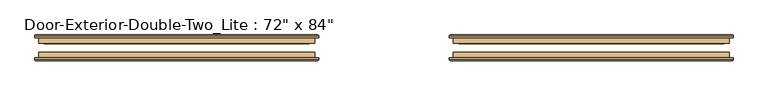
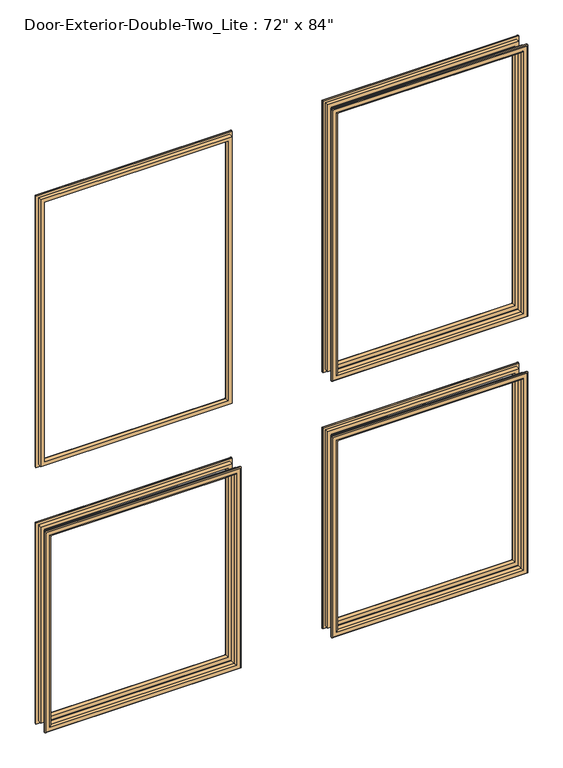
"""IFC4 building model written with IfcOpenShell, lengths in millimetres: door geometry."""

from ifc_helpers import new_model, si_unit, frame, origin, place, context, project, spatial, ellipse_curve, source, transform, mapped, element, save
from ifc_brep_helpers import plane_surface, cylinder_surface, advanced_brep


def door_5583bd1b(model_context):
    return source(origin(), model_context, "Body", "AdvancedBrep", [
        advanced_brep(
        [(-762.0, 55.5625, 914.4), (-762.0, 68.2625, 914.4), (-762.0, 68.2625, 254.0), (-762.0, 55.5625, 254.0), (-750.0, 69.2625, 902.4), (-750.0, 55.5625, 902.4), (-750.0, 55.5625, 266.0), (-750.0, 69.2625, 266.0), (-755.0, 74.2625, 907.4), (-755.0, 74.2625, 261.0), (-770.0, 72.2625, 922.4), (-768.0, 74.2625, 920.4), (-768.0, 74.2625, 248.0), (-770.0, 72.2625, 246.0), (-770.0, 68.2625, 922.4), (-770.0, 68.2625, 246.0), (-152.4, 68.2625, 254.0), (-152.4, 55.5625, 254.0), (-164.4, 55.5625, 266.0), (-164.4, 69.2625, 266.0), (-159.4, 74.2625, 261.0), (-146.4, 74.2625, 248.0), (-144.4, 72.2625, 246.0), (-144.4, 68.2625, 246.0), (-152.4, 68.2625, 914.4), (-152.4, 55.5625, 914.4), (-164.4, 55.5625, 902.4), (-164.4, 69.2625, 902.4), (-159.4, 74.2625, 907.4), (-146.4, 74.2625, 920.4), (-144.4, 72.2625, 922.4), (-144.4, 68.2625, 922.4)],
        [
            (0, 1),
            (1, 2),
            (2, 3),
            (3, 0),
            (4, 5),
            (5, 6),
            (6, 7),
            (7, 4),
            (8, 4, ellipse_curve(frame((-755.0, 69.2625, 907.4), z_axis=(-0.7071067811865475, 0.0, -0.7071067811865475), x_axis=(-0.7071067811865474, 0.0, 0.7071067811865476)), 7.0710678, 5.0)),
            (7, 9, ellipse_curve(frame((-755.0, 69.2625, 261.0), z_axis=(-0.7071067811865475, 0.0, 0.7071067811865475), x_axis=(0.7071067811865474, 0.0, 0.7071067811865476)), 7.0710678, 5.0)),
            (9, 8),
            (10, 11, ellipse_curve(frame((-768.0, 72.2625, 920.4), z_axis=(-0.7071067811865475, 0.0, -0.7071067811865475), x_axis=(-0.7071067811865474, 0.0, 0.7071067811865476)), 2.8284271, 2.0)),
            (11, 12),
            (12, 13, ellipse_curve(frame((-768.0, 72.2625, 248.0), z_axis=(-0.7071067811865475, 0.0, 0.7071067811865475), x_axis=(0.7071067811865474, 0.0, 0.7071067811865476)), 2.8284271, 2.0)),
            (13, 10),
            (14, 10),
            (13, 15),
            (15, 14),
            (2, 16),
            (16, 17),
            (17, 3),
            (6, 18),
            (18, 19),
            (19, 7),
            (19, 20, ellipse_curve(frame((-159.4, 69.2625, 261.0), z_axis=(-0.7071067811865475, 0.0, -0.7071067811865475), x_axis=(-0.7071067811865476, 0.0, 0.7071067811865474)), 7.0710678, 5.0)),
            (20, 9),
            (12, 21),
            (21, 22, ellipse_curve(frame((-146.4, 72.2625, 248.0), z_axis=(-0.7071067811865475, 0.0, -0.7071067811865475), x_axis=(-0.7071067811865476, 0.0, 0.7071067811865474)), 2.8284271, 2.0)),
            (22, 13),
            (22, 23),
            (23, 15),
            (16, 24),
            (24, 25),
            (25, 17),
            (18, 26),
            (26, 27),
            (27, 19),
            (27, 28, ellipse_curve(frame((-159.4, 69.2625, 907.4), z_axis=(0.7071067811865475, 0.0, -0.7071067811865475), x_axis=(-0.7071067811865474, 0.0, -0.7071067811865476)), 7.0710678, 5.0)),
            (28, 20),
            (21, 29),
            (29, 30, ellipse_curve(frame((-146.4, 72.2625, 920.4), z_axis=(0.7071067811865475, 0.0, -0.7071067811865475), x_axis=(-0.7071067811865474, 0.0, -0.7071067811865476)), 2.8284271, 2.0)),
            (30, 22),
            (30, 31),
            (31, 23),
            (31, 14),
            (1, 24),
            (0, 25),
            (5, 26),
            (4, 27),
            (8, 28),
            (11, 29),
            (10, 30),
        ],
        [
            plane_surface(frame((-762.0, 68.2625, 914.4), z_axis=(-1.0, 0.0, 0.0), x_axis=(0.0, 0.0, -1.0))),
            plane_surface(frame((-750.0, 55.5625, 902.4), z_axis=(1.0, 0.0, 0.0), x_axis=(0.0, 0.0, -1.0))),
            cylinder_surface(frame((-755.0, 69.2625, 914.4), z_axis=(0.0, 0.0, 1.0), x_axis=(-1.0, 0.0, 0.0)), 5.0),
            cylinder_surface(frame((-768.0, 72.2625, 914.4), z_axis=(0.0, 0.0, 1.0), x_axis=(-1.0, 0.0, 0.0)), 2.0),
            plane_surface(frame((-770.0, 72.2625, 922.4), z_axis=(-1.0, 0.0, 0.0), x_axis=(0.0, 0.0, -1.0))),
            plane_surface(frame((-762.0, 68.2625, 254.0), z_axis=(0.0, 0.0, -1.0), x_axis=(1.0, 0.0, 0.0))),
            plane_surface(frame((-750.0, 55.5625, 266.0), z_axis=(0.0, 0.0, 1.0), x_axis=(1.0, 0.0, 0.0))),
            cylinder_surface(frame((-762.0, 69.2625, 261.0), z_axis=(-1.0, 0.0, 0.0), x_axis=(0.0, 0.0, -1.0)), 5.0),
            cylinder_surface(frame((-762.0, 72.2625, 248.0), z_axis=(-1.0, 0.0, 0.0), x_axis=(0.0, 0.0, -1.0)), 2.0),
            plane_surface(frame((-770.0, 72.2625, 246.0), z_axis=(0.0, 0.0, -1.0), x_axis=(1.0, 0.0, 0.0))),
            plane_surface(frame((-152.4, 68.2625, 254.0), z_axis=(1.0, 0.0, 0.0), x_axis=(0.0, 0.0, 1.0))),
            plane_surface(frame((-164.4, 55.5625, 266.0), z_axis=(-1.0, 0.0, 0.0), x_axis=(0.0, 0.0, 1.0))),
            cylinder_surface(frame((-159.4, 69.2625, 254.0), z_axis=(0.0, 0.0, -1.0), x_axis=(1.0, 0.0, 0.0)), 5.0),
            cylinder_surface(frame((-146.4, 72.2625, 254.0), z_axis=(0.0, 0.0, -1.0), x_axis=(1.0, 0.0, 0.0)), 2.0),
            plane_surface(frame((-144.4, 72.2625, 246.0), z_axis=(1.0, 0.0, 0.0), x_axis=(0.0, 0.0, 1.0))),
            plane_surface(frame((-144.4, 68.2625, 922.4), z_axis=(0.0, -1.0, 0.0), x_axis=(-1.0, 0.0, 0.0))),
            plane_surface(frame((-152.4, 68.2625, 914.4), z_axis=(0.0, 0.0, 1.0), x_axis=(-1.0, 0.0, 0.0))),
            plane_surface(frame((-152.4, 55.5625, 914.4), z_axis=(0.0, -1.0, 0.0), x_axis=(-1.0, 0.0, 0.0))),
            plane_surface(frame((-164.4, 55.5625, 902.4), z_axis=(0.0, 0.0, -1.0), x_axis=(-1.0, 0.0, 0.0))),
            cylinder_surface(frame((-152.4, 69.2625, 907.4), z_axis=(1.0, 0.0, 0.0), x_axis=(0.0, 0.0, 1.0)), 5.0),
            plane_surface(frame((-159.4, 74.2625, 907.4), z_axis=(0.0, 1.0, 0.0), x_axis=(-1.0, 0.0, 0.0))),
            cylinder_surface(frame((-152.4, 72.2625, 920.4), z_axis=(1.0, 0.0, 0.0), x_axis=(0.0, 0.0, 1.0)), 2.0),
            plane_surface(frame((-144.4, 72.2625, 922.4), z_axis=(0.0, 0.0, 1.0), x_axis=(-1.0, 0.0, 0.0))),
        ],
        [
            (0, [[1, 2, 3, 4]]),
            (1, [[5, 6, 7, 8]]),
            (2, [[9, -8, 10, 11]]),
            (3, [[12, 13, 14, 15]]),
            (4, [[16, -15, 17, 18]]),
            (5, [[-3, 19, 20, 21]]),
            (6, [[-7, 22, 23, 24]]),
            (7, [[-10, -24, 25, 26]]),
            (8, [[-14, 27, 28, 29]]),
            (9, [[-17, -29, 30, 31]]),
            (10, [[-20, 32, 33, 34]]),
            (11, [[-23, 35, 36, 37]]),
            (12, [[-25, -37, 38, 39]]),
            (13, [[-28, 40, 41, 42]]),
            (14, [[-30, -42, 43, 44]]),
            (15, [[-31, -44, 45, -18], [46, -32, -19, -2]]),
            (16, [[-33, -46, -1, 47]]),
            (17, [[-21, -34, -47, -4], [48, -35, -22, -6]]),
            (18, [[-36, -48, -5, 49]]),
            (19, [[-38, -49, -9, 50]]),
            (20, [[51, -40, -27, -13], [-26, -39, -50, -11]]),
            (21, [[-41, -51, -12, 52]]),
            (22, [[-43, -52, -16, -45]]),
        ],
    ),
        advanced_brep(
        [(152.4, 55.5625, 914.4), (152.4, 68.2625, 914.4), (152.4, 68.2625, 254.0), (152.4, 55.5625, 254.0), (164.4, 69.2625, 902.4), (164.4, 55.5625, 902.4), (164.4, 55.5625, 266.0), (164.4, 69.2625, 266.0), (159.4, 74.2625, 907.4), (159.4, 74.2625, 261.0), (144.4, 72.2625, 922.4), (146.4, 74.2625, 920.4), (146.4, 74.2625, 248.0), (144.4, 72.2625, 246.0), (144.4, 68.2625, 922.4), (144.4, 68.2625, 246.0), (762.0, 68.2625, 254.0), (762.0, 55.5625, 254.0), (750.0, 55.5625, 266.0), (750.0, 69.2625, 266.0), (755.0, 74.2625, 261.0), (768.0, 74.2625, 248.0), (770.0, 72.2625, 246.0), (770.0, 68.2625, 246.0), (762.0, 68.2625, 914.4), (762.0, 55.5625, 914.4), (750.0, 55.5625, 902.4), (750.0, 69.2625, 902.4), (755.0, 74.2625, 907.4), (768.0, 74.2625, 920.4), (770.0, 72.2625, 922.4), (770.0, 68.2625, 922.4)],
        [
            (0, 1),
            (1, 2),
            (2, 3),
            (3, 0),
            (4, 5),
            (5, 6),
            (6, 7),
            (7, 4),
            (8, 4, ellipse_curve(frame((159.4, 69.2625, 907.4), z_axis=(-0.7071067811865475, 0.0, -0.7071067811865475), x_axis=(-0.7071067811865474, 0.0, 0.7071067811865476)), 7.0710678, 5.0)),
            (7, 9, ellipse_curve(frame((159.4, 69.2625, 261.0), z_axis=(-0.7071067811865475, 0.0, 0.7071067811865475), x_axis=(0.7071067811865474, 0.0, 0.7071067811865476)), 7.0710678, 5.0)),
            (9, 8),
            (10, 11, ellipse_curve(frame((146.4, 72.2625, 920.4), z_axis=(-0.7071067811865475, 0.0, -0.7071067811865475), x_axis=(-0.7071067811865474, 0.0, 0.7071067811865476)), 2.8284271, 2.0)),
            (11, 12),
            (12, 13, ellipse_curve(frame((146.4, 72.2625, 248.0), z_axis=(-0.7071067811865475, 0.0, 0.7071067811865475), x_axis=(0.7071067811865474, 0.0, 0.7071067811865476)), 2.8284271, 2.0)),
            (13, 10),
            (14, 10),
            (13, 15),
            (15, 14),
            (2, 16),
            (16, 17),
            (17, 3),
            (6, 18),
            (18, 19),
            (19, 7),
            (19, 20, ellipse_curve(frame((755.0, 69.2625, 261.0), z_axis=(-0.7071067811865475, 0.0, -0.7071067811865475), x_axis=(-0.7071067811865476, 0.0, 0.7071067811865474)), 7.0710678, 5.0)),
            (20, 9),
            (12, 21),
            (21, 22, ellipse_curve(frame((768.0, 72.2625, 248.0), z_axis=(-0.7071067811865475, 0.0, -0.7071067811865475), x_axis=(-0.7071067811865476, 0.0, 0.7071067811865474)), 2.8284271, 2.0)),
            (22, 13),
            (22, 23),
            (23, 15),
            (16, 24),
            (24, 25),
            (25, 17),
            (18, 26),
            (26, 27),
            (27, 19),
            (27, 28, ellipse_curve(frame((755.0, 69.2625, 907.4), z_axis=(0.7071067811865475, 0.0, -0.7071067811865475), x_axis=(-0.7071067811865474, 0.0, -0.7071067811865476)), 7.0710678, 5.0)),
            (28, 20),
            (21, 29),
            (29, 30, ellipse_curve(frame((768.0, 72.2625, 920.4), z_axis=(0.7071067811865475, 0.0, -0.7071067811865475), x_axis=(-0.7071067811865474, 0.0, -0.7071067811865476)), 2.8284271, 2.0)),
            (30, 22),
            (30, 31),
            (31, 23),
            (31, 14),
            (1, 24),
            (0, 25),
            (5, 26),
            (4, 27),
            (8, 28),
            (11, 29),
            (10, 30),
        ],
        [
            plane_surface(frame((152.4, 68.2625, 914.4), z_axis=(-1.0, 0.0, 0.0), x_axis=(0.0, 0.0, -1.0))),
            plane_surface(frame((164.4, 55.5625, 902.4), z_axis=(1.0, 0.0, 0.0), x_axis=(0.0, 0.0, -1.0))),
            cylinder_surface(frame((159.4, 69.2625, 914.4), z_axis=(0.0, 0.0, 1.0), x_axis=(-1.0, 0.0, 0.0)), 5.0),
            cylinder_surface(frame((146.4, 72.2625, 914.4), z_axis=(0.0, 0.0, 1.0), x_axis=(-1.0, 0.0, 0.0)), 2.0),
            plane_surface(frame((144.4, 72.2625, 922.4), z_axis=(-1.0, 0.0, 0.0), x_axis=(0.0, 0.0, -1.0))),
            plane_surface(frame((152.4, 68.2625, 254.0), z_axis=(0.0, 0.0, -1.0), x_axis=(1.0, 0.0, 0.0))),
            plane_surface(frame((164.4, 55.5625, 266.0), z_axis=(0.0, 0.0, 1.0), x_axis=(1.0, 0.0, 0.0))),
            cylinder_surface(frame((152.4, 69.2625, 261.0), z_axis=(-1.0, 0.0, 0.0), x_axis=(0.0, 0.0, -1.0)), 5.0),
            cylinder_surface(frame((152.4, 72.2625, 248.0), z_axis=(-1.0, 0.0, 0.0), x_axis=(0.0, 0.0, -1.0)), 2.0),
            plane_surface(frame((144.4, 72.2625, 246.0), z_axis=(0.0, 0.0, -1.0), x_axis=(1.0, 0.0, 0.0))),
            plane_surface(frame((762.0, 68.2625, 254.0), z_axis=(1.0, 0.0, 0.0), x_axis=(0.0, 0.0, 1.0))),
            plane_surface(frame((750.0, 55.5625, 266.0), z_axis=(-1.0, 0.0, 0.0), x_axis=(0.0, 0.0, 1.0))),
            cylinder_surface(frame((755.0, 69.2625, 254.0), z_axis=(0.0, 0.0, -1.0), x_axis=(1.0, 0.0, 0.0)), 5.0),
            cylinder_surface(frame((768.0, 72.2625, 254.0), z_axis=(0.0, 0.0, -1.0), x_axis=(1.0, 0.0, 0.0)), 2.0),
            plane_surface(frame((770.0, 72.2625, 246.0), z_axis=(1.0, 0.0, 0.0), x_axis=(0.0, 0.0, 1.0))),
            plane_surface(frame((770.0, 68.2625, 922.4), z_axis=(0.0, -1.0, 0.0), x_axis=(-1.0, 0.0, 0.0))),
            plane_surface(frame((762.0, 68.2625, 914.4), z_axis=(0.0, 0.0, 1.0), x_axis=(-1.0, 0.0, 0.0))),
            plane_surface(frame((762.0, 55.5625, 914.4), z_axis=(0.0, -1.0, 0.0), x_axis=(-1.0, 0.0, 0.0))),
            plane_surface(frame((750.0, 55.5625, 902.4), z_axis=(0.0, 0.0, -1.0), x_axis=(-1.0, 0.0, 0.0))),
            cylinder_surface(frame((762.0, 69.2625, 907.4), z_axis=(1.0, 0.0, 0.0), x_axis=(0.0, 0.0, 1.0)), 5.0),
            plane_surface(frame((755.0, 74.2625, 907.4), z_axis=(0.0, 1.0, 0.0), x_axis=(-1.0, 0.0, 0.0))),
            cylinder_surface(frame((762.0, 72.2625, 920.4), z_axis=(1.0, 0.0, 0.0), x_axis=(0.0, 0.0, 1.0)), 2.0),
            plane_surface(frame((770.0, 72.2625, 922.4), z_axis=(0.0, 0.0, 1.0), x_axis=(-1.0, 0.0, 0.0))),
        ],
        [
            (0, [[1, 2, 3, 4]]),
            (1, [[5, 6, 7, 8]]),
            (2, [[9, -8, 10, 11]]),
            (3, [[12, 13, 14, 15]]),
            (4, [[16, -15, 17, 18]]),
            (5, [[-3, 19, 20, 21]]),
            (6, [[-7, 22, 23, 24]]),
            (7, [[-10, -24, 25, 26]]),
            (8, [[-14, 27, 28, 29]]),
            (9, [[-17, -29, 30, 31]]),
            (10, [[-20, 32, 33, 34]]),
            (11, [[-23, 35, 36, 37]]),
            (12, [[-25, -37, 38, 39]]),
            (13, [[-28, 40, 41, 42]]),
            (14, [[-30, -42, 43, 44]]),
            (15, [[-31, -44, 45, -18], [46, -32, -19, -2]]),
            (16, [[-33, -46, -1, 47]]),
            (17, [[-21, -34, -47, -4], [48, -35, -22, -6]]),
            (18, [[-36, -48, -5, 49]]),
            (19, [[-38, -49, -9, 50]]),
            (20, [[51, -40, -27, -13], [-26, -39, -50, -11]]),
            (21, [[-41, -51, -12, 52]]),
            (22, [[-43, -52, -16, -45]]),
        ],
    ),
        advanced_brep(
        [(152.4, 55.5625, 2016.125), (152.4, 68.2625, 2016.125), (152.4, 68.2625, 1117.6), (152.4, 55.5625, 1117.6), (164.4, 69.2625, 2004.125), (164.4, 55.5625, 2004.125), (164.4, 55.5625, 1129.6), (164.4, 69.2625, 1129.6), (159.4, 74.2625, 2009.125), (159.4, 74.2625, 1124.6), (144.4, 72.2625, 2024.125), (146.4, 74.2625, 2022.125), (146.4, 74.2625, 1111.6), (144.4, 72.2625, 1109.6), (144.4, 68.2625, 2024.125), (144.4, 68.2625, 1109.6), (762.0, 68.2625, 1117.6), (762.0, 55.5625, 1117.6), (750.0, 55.5625, 1129.6), (750.0, 69.2625, 1129.6), (755.0, 74.2625, 1124.6), (768.0, 74.2625, 1111.6), (770.0, 72.2625, 1109.6), (770.0, 68.2625, 1109.6), (762.0, 68.2625, 2016.125), (762.0, 55.5625, 2016.125), (750.0, 55.5625, 2004.125), (750.0, 69.2625, 2004.125), (755.0, 74.2625, 2009.125), (768.0, 74.2625, 2022.125), (770.0, 72.2625, 2024.125), (770.0, 68.2625, 2024.125)],
        [
            (0, 1),
            (1, 2),
            (2, 3),
            (3, 0),
            (4, 5),
            (5, 6),
            (6, 7),
            (7, 4),
            (8, 4, ellipse_curve(frame((159.4, 69.2625, 2009.125), z_axis=(-0.7071067811865475, 0.0, -0.7071067811865475), x_axis=(-0.7071067811865474, 0.0, 0.7071067811865476)), 7.0710678, 5.0)),
            (7, 9, ellipse_curve(frame((159.4, 69.2625, 1124.6), z_axis=(-0.7071067811865475, 0.0, 0.7071067811865475), x_axis=(0.7071067811865474, 0.0, 0.7071067811865476)), 7.0710678, 5.0)),
            (9, 8),
            (10, 11, ellipse_curve(frame((146.4, 72.2625, 2022.125), z_axis=(-0.7071067811865475, 0.0, -0.7071067811865475), x_axis=(-0.7071067811865474, 0.0, 0.7071067811865476)), 2.8284271, 2.0)),
            (11, 12),
            (12, 13, ellipse_curve(frame((146.4, 72.2625, 1111.6), z_axis=(-0.7071067811865475, 0.0, 0.7071067811865475), x_axis=(0.7071067811865474, 0.0, 0.7071067811865476)), 2.8284271, 2.0)),
            (13, 10),
            (14, 10),
            (13, 15),
            (15, 14),
            (2, 16),
            (16, 17),
            (17, 3),
            (6, 18),
            (18, 19),
            (19, 7),
            (19, 20, ellipse_curve(frame((755.0, 69.2625, 1124.6), z_axis=(-0.7071067811865475, 0.0, -0.7071067811865475), x_axis=(-0.7071067811865476, 0.0, 0.7071067811865474)), 7.0710678, 5.0)),
            (20, 9),
            (12, 21),
            (21, 22, ellipse_curve(frame((768.0, 72.2625, 1111.6), z_axis=(-0.7071067811865475, 0.0, -0.7071067811865475), x_axis=(-0.7071067811865476, 0.0, 0.7071067811865474)), 2.8284271, 2.0)),
            (22, 13),
            (22, 23),
            (23, 15),
            (16, 24),
            (24, 25),
            (25, 17),
            (18, 26),
            (26, 27),
            (27, 19),
            (27, 28, ellipse_curve(frame((755.0, 69.2625, 2009.125), z_axis=(0.7071067811865475, 0.0, -0.7071067811865475), x_axis=(-0.7071067811865474, 0.0, -0.7071067811865476)), 7.0710678, 5.0)),
            (28, 20),
            (21, 29),
            (29, 30, ellipse_curve(frame((768.0, 72.2625, 2022.125), z_axis=(0.7071067811865475, 0.0, -0.7071067811865475), x_axis=(-0.7071067811865474, 0.0, -0.7071067811865476)), 2.8284271, 2.0)),
            (30, 22),
            (30, 31),
            (31, 23),
            (31, 14),
            (1, 24),
            (0, 25),
            (5, 26),
            (4, 27),
            (8, 28),
            (11, 29),
            (10, 30),
        ],
        [
            plane_surface(frame((152.4, 68.2625, 2016.125), z_axis=(-1.0, 0.0, 0.0), x_axis=(0.0, 0.0, -1.0))),
            plane_surface(frame((164.4, 55.5625, 2004.125), z_axis=(1.0, 0.0, 0.0), x_axis=(0.0, 0.0, -1.0))),
            cylinder_surface(frame((159.4, 69.2625, 2016.125), z_axis=(0.0, 0.0, 1.0), x_axis=(-1.0, 0.0, 0.0)), 5.0),
            cylinder_surface(frame((146.4, 72.2625, 2016.125), z_axis=(0.0, 0.0, 1.0), x_axis=(-1.0, 0.0, 0.0)), 2.0),
            plane_surface(frame((144.4, 72.2625, 2024.125), z_axis=(-1.0, 0.0, 0.0), x_axis=(0.0, 0.0, -1.0))),
            plane_surface(frame((152.4, 68.2625, 1117.6), z_axis=(0.0, 0.0, -1.0), x_axis=(1.0, 0.0, 0.0))),
            plane_surface(frame((164.4, 55.5625, 1129.6), z_axis=(0.0, 0.0, 1.0), x_axis=(1.0, 0.0, 0.0))),
            cylinder_surface(frame((152.4, 69.2625, 1124.6), z_axis=(-1.0, 0.0, 0.0), x_axis=(0.0, 0.0, -1.0)), 5.0),
            cylinder_surface(frame((152.4, 72.2625, 1111.6), z_axis=(-1.0, 0.0, 0.0), x_axis=(0.0, 0.0, -1.0)), 2.0),
            plane_surface(frame((144.4, 72.2625, 1109.6), z_axis=(0.0, 0.0, -1.0), x_axis=(1.0, 0.0, 0.0))),
            plane_surface(frame((762.0, 68.2625, 1117.6), z_axis=(1.0, 0.0, 0.0), x_axis=(0.0, 0.0, 1.0))),
            plane_surface(frame((750.0, 55.5625, 1129.6), z_axis=(-1.0, 0.0, 0.0), x_axis=(0.0, 0.0, 1.0))),
            cylinder_surface(frame((755.0, 69.2625, 1117.6), z_axis=(0.0, 0.0, -1.0), x_axis=(1.0, 0.0, 0.0)), 5.0),
            cylinder_surface(frame((768.0, 72.2625, 1117.6), z_axis=(0.0, 0.0, -1.0), x_axis=(1.0, 0.0, 0.0)), 2.0),
            plane_surface(frame((770.0, 72.2625, 1109.6), z_axis=(1.0, 0.0, 0.0), x_axis=(0.0, 0.0, 1.0))),
            plane_surface(frame((770.0, 68.2625, 2024.125), z_axis=(0.0, -1.0, 0.0), x_axis=(-1.0, 0.0, 0.0))),
            plane_surface(frame((762.0, 68.2625, 2016.125), z_axis=(0.0, 0.0, 1.0), x_axis=(-1.0, 0.0, 0.0))),
            plane_surface(frame((762.0, 55.5625, 2016.125), z_axis=(0.0, -1.0, 0.0), x_axis=(-1.0, 0.0, 0.0))),
            plane_surface(frame((750.0, 55.5625, 2004.125), z_axis=(0.0, 0.0, -1.0), x_axis=(-1.0, 0.0, 0.0))),
            cylinder_surface(frame((762.0, 69.2625, 2009.125), z_axis=(1.0, 0.0, 0.0), x_axis=(0.0, 0.0, 1.0)), 5.0),
            plane_surface(frame((755.0, 74.2625, 2009.125), z_axis=(0.0, 1.0, 0.0), x_axis=(-1.0, 0.0, 0.0))),
            cylinder_surface(frame((762.0, 72.2625, 2022.125), z_axis=(1.0, 0.0, 0.0), x_axis=(0.0, 0.0, 1.0)), 2.0),
            plane_surface(frame((770.0, 72.2625, 2024.125), z_axis=(0.0, 0.0, 1.0), x_axis=(-1.0, 0.0, 0.0))),
        ],
        [
            (0, [[1, 2, 3, 4]]),
            (1, [[5, 6, 7, 8]]),
            (2, [[9, -8, 10, 11]]),
            (3, [[12, 13, 14, 15]]),
            (4, [[16, -15, 17, 18]]),
            (5, [[-3, 19, 20, 21]]),
            (6, [[-7, 22, 23, 24]]),
            (7, [[-10, -24, 25, 26]]),
            (8, [[-14, 27, 28, 29]]),
            (9, [[-17, -29, 30, 31]]),
            (10, [[-20, 32, 33, 34]]),
            (11, [[-23, 35, 36, 37]]),
            (12, [[-25, -37, 38, 39]]),
            (13, [[-28, 40, 41, 42]]),
            (14, [[-30, -42, 43, 44]]),
            (15, [[-31, -44, 45, -18], [46, -32, -19, -2]]),
            (16, [[-33, -46, -1, 47]]),
            (17, [[-21, -34, -47, -4], [48, -35, -22, -6]]),
            (18, [[-36, -48, -5, 49]]),
            (19, [[-38, -49, -9, 50]]),
            (20, [[51, -40, -27, -13], [-26, -39, -50, -11]]),
            (21, [[-41, -51, -12, 52]]),
            (22, [[-43, -52, -16, -45]]),
        ],
    ),
        advanced_brep(
        [(-762.0, 55.5625, 2016.125), (-762.0, 68.2625, 2016.125), (-762.0, 68.2625, 1117.6), (-762.0, 55.5625, 1117.6), (-750.0, 69.2625, 2004.125), (-750.0, 55.5625, 2004.125), (-750.0, 55.5625, 1129.6), (-750.0, 69.2625, 1129.6), (-755.0, 74.2625, 2009.125), (-755.0, 74.2625, 1124.6), (-770.0, 72.2625, 2024.125), (-768.0, 74.2625, 2022.125), (-768.0, 74.2625, 1111.6), (-770.0, 72.2625, 1109.6), (-770.0, 68.2625, 2024.125), (-770.0, 68.2625, 1109.6), (-152.4, 68.2625, 1117.6), (-152.4, 55.5625, 1117.6), (-164.4, 55.5625, 1129.6), (-164.4, 69.2625, 1129.6), (-159.4, 74.2625, 1124.6), (-146.4, 74.2625, 1111.6), (-144.4, 72.2625, 1109.6), (-144.4, 68.2625, 1109.6), (-152.4, 68.2625, 2016.125), (-152.4, 55.5625, 2016.125), (-164.4, 55.5625, 2004.125), (-164.4, 69.2625, 2004.125), (-159.4, 74.2625, 2009.125), (-146.4, 74.2625, 2022.125), (-144.4, 72.2625, 2024.125), (-144.4, 68.2625, 2024.125)],
        [
            (0, 1),
            (1, 2),
            (2, 3),
            (3, 0),
            (4, 5),
            (5, 6),
            (6, 7),
            (7, 4),
            (8, 4, ellipse_curve(frame((-755.0, 69.2625, 2009.125), z_axis=(-0.7071067811865475, 0.0, -0.7071067811865475), x_axis=(-0.7071067811865474, 0.0, 0.7071067811865476)), 7.0710678, 5.0)),
            (7, 9, ellipse_curve(frame((-755.0, 69.2625, 1124.6), z_axis=(-0.7071067811865475, 0.0, 0.7071067811865475), x_axis=(0.7071067811865474, 0.0, 0.7071067811865476)), 7.0710678, 5.0)),
            (9, 8),
            (10, 11, ellipse_curve(frame((-768.0, 72.2625, 2022.125), z_axis=(-0.7071067811865475, 0.0, -0.7071067811865475), x_axis=(-0.7071067811865474, 0.0, 0.7071067811865476)), 2.8284271, 2.0)),
            (11, 12),
            (12, 13, ellipse_curve(frame((-768.0, 72.2625, 1111.6), z_axis=(-0.7071067811865475, 0.0, 0.7071067811865475), x_axis=(0.7071067811865474, 0.0, 0.7071067811865476)), 2.8284271, 2.0)),
            (13, 10),
            (14, 10),
            (13, 15),
            (15, 14),
            (2, 16),
            (16, 17),
            (17, 3),
            (6, 18),
            (18, 19),
            (19, 7),
            (19, 20, ellipse_curve(frame((-159.4, 69.2625, 1124.6), z_axis=(-0.7071067811865475, 0.0, -0.7071067811865475), x_axis=(-0.7071067811865476, 0.0, 0.7071067811865474)), 7.0710678, 5.0)),
            (20, 9),
            (12, 21),
            (21, 22, ellipse_curve(frame((-146.4, 72.2625, 1111.6), z_axis=(-0.7071067811865475, 0.0, -0.7071067811865475), x_axis=(-0.7071067811865476, 0.0, 0.7071067811865474)), 2.8284271, 2.0)),
            (22, 13),
            (22, 23),
            (23, 15),
            (16, 24),
            (24, 25),
            (25, 17),
            (18, 26),
            (26, 27),
            (27, 19),
            (27, 28, ellipse_curve(frame((-159.4, 69.2625, 2009.125), z_axis=(0.7071067811865475, 0.0, -0.7071067811865475), x_axis=(-0.7071067811865474, 0.0, -0.7071067811865476)), 7.0710678, 5.0)),
            (28, 20),
            (21, 29),
            (29, 30, ellipse_curve(frame((-146.4, 72.2625, 2022.125), z_axis=(0.7071067811865475, 0.0, -0.7071067811865475), x_axis=(-0.7071067811865474, 0.0, -0.7071067811865476)), 2.8284271, 2.0)),
            (30, 22),
            (30, 31),
            (31, 23),
            (31, 14),
            (1, 24),
            (0, 25),
            (5, 26),
            (4, 27),
            (8, 28),
            (11, 29),
            (10, 30),
        ],
        [
            plane_surface(frame((-762.0, 68.2625, 2016.125), z_axis=(-1.0, 0.0, 0.0), x_axis=(0.0, 0.0, -1.0))),
            plane_surface(frame((-750.0, 55.5625, 2004.125), z_axis=(1.0, 0.0, 0.0), x_axis=(0.0, 0.0, -1.0))),
            cylinder_surface(frame((-755.0, 69.2625, 2016.125), z_axis=(0.0, 0.0, 1.0), x_axis=(-1.0, 0.0, 0.0)), 5.0),
            cylinder_surface(frame((-768.0, 72.2625, 2016.125), z_axis=(0.0, 0.0, 1.0), x_axis=(-1.0, 0.0, 0.0)), 2.0),
            plane_surface(frame((-770.0, 72.2625, 2024.125), z_axis=(-1.0, 0.0, 0.0), x_axis=(0.0, 0.0, -1.0))),
            plane_surface(frame((-762.0, 68.2625, 1117.6), z_axis=(0.0, 0.0, -1.0), x_axis=(1.0, 0.0, 0.0))),
            plane_surface(frame((-750.0, 55.5625, 1129.6), z_axis=(0.0, 0.0, 1.0), x_axis=(1.0, 0.0, 0.0))),
            cylinder_surface(frame((-762.0, 69.2625, 1124.6), z_axis=(-1.0, 0.0, 0.0), x_axis=(0.0, 0.0, -1.0)), 5.0),
            cylinder_surface(frame((-762.0, 72.2625, 1111.6), z_axis=(-1.0, 0.0, 0.0), x_axis=(0.0, 0.0, -1.0)), 2.0),
            plane_surface(frame((-770.0, 72.2625, 1109.6), z_axis=(0.0, 0.0, -1.0), x_axis=(1.0, 0.0, 0.0))),
            plane_surface(frame((-152.4, 68.2625, 1117.6), z_axis=(1.0, 0.0, 0.0), x_axis=(0.0, 0.0, 1.0))),
            plane_surface(frame((-164.4, 55.5625, 1129.6), z_axis=(-1.0, 0.0, 0.0), x_axis=(0.0, 0.0, 1.0))),
            cylinder_surface(frame((-159.4, 69.2625, 1117.6), z_axis=(0.0, 0.0, -1.0), x_axis=(1.0, 0.0, 0.0)), 5.0),
            cylinder_surface(frame((-146.4, 72.2625, 1117.6), z_axis=(0.0, 0.0, -1.0), x_axis=(1.0, 0.0, 0.0)), 2.0),
            plane_surface(frame((-144.4, 72.2625, 1109.6), z_axis=(1.0, 0.0, 0.0), x_axis=(0.0, 0.0, 1.0))),
            plane_surface(frame((-144.4, 68.2625, 2024.125), z_axis=(0.0, -1.0, 0.0), x_axis=(-1.0, 0.0, 0.0))),
            plane_surface(frame((-152.4, 68.2625, 2016.125), z_axis=(0.0, 0.0, 1.0), x_axis=(-1.0, 0.0, 0.0))),
            plane_surface(frame((-152.4, 55.5625, 2016.125), z_axis=(0.0, -1.0, 0.0), x_axis=(-1.0, 0.0, 0.0))),
            plane_surface(frame((-164.4, 55.5625, 2004.125), z_axis=(0.0, 0.0, -1.0), x_axis=(-1.0, 0.0, 0.0))),
            cylinder_surface(frame((-152.4, 69.2625, 2009.125), z_axis=(1.0, 0.0, 0.0), x_axis=(0.0, 0.0, 1.0)), 5.0),
            plane_surface(frame((-159.4, 74.2625, 2009.125), z_axis=(0.0, 1.0, 0.0), x_axis=(-1.0, 0.0, 0.0))),
            cylinder_surface(frame((-152.4, 72.2625, 2022.125), z_axis=(1.0, 0.0, 0.0), x_axis=(0.0, 0.0, 1.0)), 2.0),
            plane_surface(frame((-144.4, 72.2625, 2024.125), z_axis=(0.0, 0.0, 1.0), x_axis=(-1.0, 0.0, 0.0))),
        ],
        [
            (0, [[1, 2, 3, 4]]),
            (1, [[5, 6, 7, 8]]),
            (2, [[9, -8, 10, 11]]),
            (3, [[12, 13, 14, 15]]),
            (4, [[16, -15, 17, 18]]),
            (5, [[-3, 19, 20, 21]]),
            (6, [[-7, 22, 23, 24]]),
            (7, [[-10, -24, 25, 26]]),
            (8, [[-14, 27, 28, 29]]),
            (9, [[-17, -29, 30, 31]]),
            (10, [[-20, 32, 33, 34]]),
            (11, [[-23, 35, 36, 37]]),
            (12, [[-25, -37, 38, 39]]),
            (13, [[-28, 40, 41, 42]]),
            (14, [[-30, -42, 43, 44]]),
            (15, [[-31, -44, 45, -18], [46, -32, -19, -2]]),
            (16, [[-33, -46, -1, 47]]),
            (17, [[-21, -34, -47, -4], [48, -35, -22, -6]]),
            (18, [[-36, -48, -5, 49]]),
            (19, [[-38, -49, -9, 50]]),
            (20, [[51, -40, -27, -13], [-26, -39, -50, -11]]),
            (21, [[-41, -51, -12, 52]]),
            (22, [[-43, -52, -16, -45]]),
        ],
    ),
        advanced_brep(
        [(-762.0, 36.5125, 254.0), (-762.0, 23.8125, 254.0), (-762.0, 23.8125, 914.4), (-762.0, 36.5125, 914.4), (-750.0, 22.8125, 266.0), (-750.0, 36.5125, 266.0), (-750.0, 36.5125, 902.4), (-750.0, 22.8125, 902.4), (-755.0, 17.8125, 261.0), (-755.0, 17.8125, 907.4), (-770.0, 19.8125, 246.0), (-768.0, 17.8125, 248.0), (-768.0, 17.8125, 920.4), (-770.0, 19.8125, 922.4), (-770.0, 23.8125, 246.0), (-770.0, 23.8125, 922.4), (-152.4, 23.8125, 914.4), (-152.4, 36.5125, 914.4), (-164.4, 36.5125, 902.4), (-164.4, 22.8125, 902.4), (-159.4, 17.8125, 907.4), (-146.4, 17.8125, 920.4), (-144.4, 19.8125, 922.4), (-144.4, 23.8125, 922.4), (-152.4, 23.8125, 254.0), (-152.4, 36.5125, 254.0), (-164.4, 36.5125, 266.0), (-164.4, 22.8125, 266.0), (-159.4, 17.8125, 261.0), (-146.4, 17.8125, 248.0), (-144.4, 19.8125, 246.0), (-144.4, 23.8125, 246.0)],
        [
            (0, 1),
            (1, 2),
            (2, 3),
            (3, 0),
            (4, 5),
            (5, 6),
            (6, 7),
            (7, 4),
            (8, 4, ellipse_curve(frame((-755.0, 22.8125, 261.0), z_axis=(-0.7071067811865475, 0.0, 0.7071067811865475), x_axis=(-0.7071067811865474, 0.0, -0.7071067811865476)), 7.0710678, 5.0)),
            (7, 9, ellipse_curve(frame((-755.0, 22.8125, 907.4), z_axis=(-0.7071067811865475, 0.0, -0.7071067811865475), x_axis=(0.7071067811865474, 0.0, -0.7071067811865476)), 7.0710678, 5.0)),
            (9, 8),
            (10, 11, ellipse_curve(frame((-768.0, 19.8125, 248.0), z_axis=(-0.7071067811865475, 0.0, 0.7071067811865475), x_axis=(-0.7071067811865474, 0.0, -0.7071067811865476)), 2.8284271, 2.0)),
            (11, 12),
            (12, 13, ellipse_curve(frame((-768.0, 19.8125, 920.4), z_axis=(-0.7071067811865475, 0.0, -0.7071067811865475), x_axis=(0.7071067811865474, 0.0, -0.7071067811865476)), 2.8284271, 2.0)),
            (13, 10),
            (14, 10),
            (13, 15),
            (15, 14),
            (2, 16),
            (16, 17),
            (17, 3),
            (6, 18),
            (18, 19),
            (19, 7),
            (19, 20, ellipse_curve(frame((-159.4, 22.8125, 907.4), z_axis=(-0.7071067811865475, 0.0, 0.7071067811865475), x_axis=(-0.7071067811865476, 0.0, -0.7071067811865474)), 7.0710678, 5.0)),
            (20, 9),
            (12, 21),
            (21, 22, ellipse_curve(frame((-146.4, 19.8125, 920.4), z_axis=(-0.7071067811865475, 0.0, 0.7071067811865475), x_axis=(-0.7071067811865476, 0.0, -0.7071067811865474)), 2.8284271, 2.0)),
            (22, 13),
            (22, 23),
            (23, 15),
            (16, 24),
            (24, 25),
            (25, 17),
            (18, 26),
            (26, 27),
            (27, 19),
            (27, 28, ellipse_curve(frame((-159.4, 22.8125, 261.0), z_axis=(0.7071067811865475, 0.0, 0.7071067811865475), x_axis=(-0.7071067811865474, 0.0, 0.7071067811865476)), 7.0710678, 5.0)),
            (28, 20),
            (21, 29),
            (29, 30, ellipse_curve(frame((-146.4, 19.8125, 248.0), z_axis=(0.7071067811865475, 0.0, 0.7071067811865475), x_axis=(-0.7071067811865474, 0.0, 0.7071067811865476)), 2.8284271, 2.0)),
            (30, 22),
            (30, 31),
            (31, 23),
            (31, 14),
            (1, 24),
            (0, 25),
            (5, 26),
            (4, 27),
            (8, 28),
            (11, 29),
            (10, 30),
        ],
        [
            plane_surface(frame((-762.0, 23.8125, 254.0), z_axis=(-1.0, 0.0, 0.0), x_axis=(0.0, 0.0, 1.0))),
            plane_surface(frame((-750.0, 36.5125, 266.0), z_axis=(1.0, 0.0, 0.0), x_axis=(0.0, 0.0, 1.0))),
            cylinder_surface(frame((-755.0, 22.8125, 254.0), z_axis=(0.0, 0.0, -1.0), x_axis=(-1.0, 0.0, 0.0)), 5.0),
            cylinder_surface(frame((-768.0, 19.8125, 254.0), z_axis=(0.0, 0.0, -1.0), x_axis=(-1.0, 0.0, 0.0)), 2.0),
            plane_surface(frame((-770.0, 19.8125, 246.0), z_axis=(-1.0, 0.0, 0.0), x_axis=(0.0, 0.0, 1.0))),
            plane_surface(frame((-762.0, 23.8125, 914.4), z_axis=(0.0, 0.0, 1.0), x_axis=(1.0, 0.0, 0.0))),
            plane_surface(frame((-750.0, 36.5125, 902.4), z_axis=(0.0, 0.0, -1.0), x_axis=(1.0, 0.0, 0.0))),
            cylinder_surface(frame((-762.0, 22.8125, 907.4), z_axis=(-1.0, 0.0, 0.0), x_axis=(0.0, 0.0, 1.0)), 5.0),
            cylinder_surface(frame((-762.0, 19.8125, 920.4), z_axis=(-1.0, 0.0, 0.0), x_axis=(0.0, 0.0, 1.0)), 2.0),
            plane_surface(frame((-770.0, 19.8125, 922.4), z_axis=(0.0, 0.0, 1.0), x_axis=(1.0, 0.0, 0.0))),
            plane_surface(frame((-152.4, 23.8125, 914.4), z_axis=(1.0, 0.0, 0.0), x_axis=(0.0, 0.0, -1.0))),
            plane_surface(frame((-164.4, 36.5125, 902.4), z_axis=(-1.0, 0.0, 0.0), x_axis=(0.0, 0.0, -1.0))),
            cylinder_surface(frame((-159.4, 22.8125, 914.4), z_axis=(0.0, 0.0, 1.0), x_axis=(1.0, 0.0, 0.0)), 5.0),
            cylinder_surface(frame((-146.4, 19.8125, 914.4), z_axis=(0.0, 0.0, 1.0), x_axis=(1.0, 0.0, 0.0)), 2.0),
            plane_surface(frame((-144.4, 19.8125, 922.4), z_axis=(1.0, 0.0, 0.0), x_axis=(0.0, 0.0, -1.0))),
            plane_surface(frame((-144.4, 23.8125, 246.0), z_axis=(0.0, 1.0, 0.0), x_axis=(-1.0, 0.0, 0.0))),
            plane_surface(frame((-152.4, 23.8125, 254.0), z_axis=(0.0, 0.0, -1.0), x_axis=(-1.0, 0.0, 0.0))),
            plane_surface(frame((-152.4, 36.5125, 254.0), z_axis=(0.0, 1.0, 0.0), x_axis=(-1.0, 0.0, 0.0))),
            plane_surface(frame((-164.4, 36.5125, 266.0), z_axis=(0.0, 0.0, 1.0), x_axis=(-1.0, 0.0, 0.0))),
            cylinder_surface(frame((-152.4, 22.8125, 261.0), z_axis=(1.0, 0.0, 0.0), x_axis=(0.0, 0.0, -1.0)), 5.0),
            plane_surface(frame((-159.4, 17.8125, 261.0), z_axis=(0.0, -1.0, 0.0), x_axis=(-1.0, 0.0, 0.0))),
            cylinder_surface(frame((-152.4, 19.8125, 248.0), z_axis=(1.0, 0.0, 0.0), x_axis=(0.0, 0.0, -1.0)), 2.0),
            plane_surface(frame((-144.4, 19.8125, 246.0), z_axis=(0.0, 0.0, -1.0), x_axis=(-1.0, 0.0, 0.0))),
        ],
        [
            (0, [[1, 2, 3, 4]]),
            (1, [[5, 6, 7, 8]]),
            (2, [[9, -8, 10, 11]]),
            (3, [[12, 13, 14, 15]]),
            (4, [[16, -15, 17, 18]]),
            (5, [[-3, 19, 20, 21]]),
            (6, [[-7, 22, 23, 24]]),
            (7, [[-10, -24, 25, 26]]),
            (8, [[-14, 27, 28, 29]]),
            (9, [[-17, -29, 30, 31]]),
            (10, [[-20, 32, 33, 34]]),
            (11, [[-23, 35, 36, 37]]),
            (12, [[-25, -37, 38, 39]]),
            (13, [[-28, 40, 41, 42]]),
            (14, [[-30, -42, 43, 44]]),
            (15, [[-31, -44, 45, -18], [46, -32, -19, -2]]),
            (16, [[-33, -46, -1, 47]]),
            (17, [[-21, -34, -47, -4], [48, -35, -22, -6]]),
            (18, [[-36, -48, -5, 49]]),
            (19, [[-38, -49, -9, 50]]),
            (20, [[51, -40, -27, -13], [-26, -39, -50, -11]]),
            (21, [[-41, -51, -12, 52]]),
            (22, [[-43, -52, -16, -45]]),
        ],
    ),
        advanced_brep(
        [(152.4, 36.5125, 254.0), (152.4, 23.8125, 254.0), (152.4, 23.8125, 914.4), (152.4, 36.5125, 914.4), (164.4, 22.8125, 266.0), (164.4, 36.5125, 266.0), (164.4, 36.5125, 902.4), (164.4, 22.8125, 902.4), (159.4, 17.8125, 261.0), (159.4, 17.8125, 907.4), (144.4, 19.8125, 246.0), (146.4, 17.8125, 248.0), (146.4, 17.8125, 920.4), (144.4, 19.8125, 922.4), (144.4, 23.8125, 246.0), (144.4, 23.8125, 922.4), (762.0, 23.8125, 914.4), (762.0, 36.5125, 914.4), (750.0, 36.5125, 902.4), (750.0, 22.8125, 902.4), (755.0, 17.8125, 907.4), (768.0, 17.8125, 920.4), (770.0, 19.8125, 922.4), (770.0, 23.8125, 922.4), (762.0, 23.8125, 254.0), (762.0, 36.5125, 254.0), (750.0, 36.5125, 266.0), (750.0, 22.8125, 266.0), (755.0, 17.8125, 261.0), (768.0, 17.8125, 248.0), (770.0, 19.8125, 246.0), (770.0, 23.8125, 246.0)],
        [
            (0, 1),
            (1, 2),
            (2, 3),
            (3, 0),
            (4, 5),
            (5, 6),
            (6, 7),
            (7, 4),
            (8, 4, ellipse_curve(frame((159.4, 22.8125, 261.0), z_axis=(-0.7071067811865475, 0.0, 0.7071067811865475), x_axis=(-0.7071067811865474, 0.0, -0.7071067811865476)), 7.0710678, 5.0)),
            (7, 9, ellipse_curve(frame((159.4, 22.8125, 907.4), z_axis=(-0.7071067811865475, 0.0, -0.7071067811865475), x_axis=(0.7071067811865474, 0.0, -0.7071067811865476)), 7.0710678, 5.0)),
            (9, 8),
            (10, 11, ellipse_curve(frame((146.4, 19.8125, 248.0), z_axis=(-0.7071067811865475, 0.0, 0.7071067811865475), x_axis=(-0.7071067811865474, 0.0, -0.7071067811865476)), 2.8284271, 2.0)),
            (11, 12),
            (12, 13, ellipse_curve(frame((146.4, 19.8125, 920.4), z_axis=(-0.7071067811865475, 0.0, -0.7071067811865475), x_axis=(0.7071067811865474, 0.0, -0.7071067811865476)), 2.8284271, 2.0)),
            (13, 10),
            (14, 10),
            (13, 15),
            (15, 14),
            (2, 16),
            (16, 17),
            (17, 3),
            (6, 18),
            (18, 19),
            (19, 7),
            (19, 20, ellipse_curve(frame((755.0, 22.8125, 907.4), z_axis=(-0.7071067811865475, 0.0, 0.7071067811865475), x_axis=(-0.7071067811865476, 0.0, -0.7071067811865474)), 7.0710678, 5.0)),
            (20, 9),
            (12, 21),
            (21, 22, ellipse_curve(frame((768.0, 19.8125, 920.4), z_axis=(-0.7071067811865475, 0.0, 0.7071067811865475), x_axis=(-0.7071067811865476, 0.0, -0.7071067811865474)), 2.8284271, 2.0)),
            (22, 13),
            (22, 23),
            (23, 15),
            (16, 24),
            (24, 25),
            (25, 17),
            (18, 26),
            (26, 27),
            (27, 19),
            (27, 28, ellipse_curve(frame((755.0, 22.8125, 261.0), z_axis=(0.7071067811865475, 0.0, 0.7071067811865475), x_axis=(-0.7071067811865474, 0.0, 0.7071067811865476)), 7.0710678, 5.0)),
            (28, 20),
            (21, 29),
            (29, 30, ellipse_curve(frame((768.0, 19.8125, 248.0), z_axis=(0.7071067811865475, 0.0, 0.7071067811865475), x_axis=(-0.7071067811865474, 0.0, 0.7071067811865476)), 2.8284271, 2.0)),
            (30, 22),
            (30, 31),
            (31, 23),
            (31, 14),
            (1, 24),
            (0, 25),
            (5, 26),
            (4, 27),
            (8, 28),
            (11, 29),
            (10, 30),
        ],
        [
            plane_surface(frame((152.4, 23.8125, 254.0), z_axis=(-1.0, 0.0, 0.0), x_axis=(0.0, 0.0, 1.0))),
            plane_surface(frame((164.4, 36.5125, 266.0), z_axis=(1.0, 0.0, 0.0), x_axis=(0.0, 0.0, 1.0))),
            cylinder_surface(frame((159.4, 22.8125, 254.0), z_axis=(0.0, 0.0, -1.0), x_axis=(-1.0, 0.0, 0.0)), 5.0),
            cylinder_surface(frame((146.4, 19.8125, 254.0), z_axis=(0.0, 0.0, -1.0), x_axis=(-1.0, 0.0, 0.0)), 2.0),
            plane_surface(frame((144.4, 19.8125, 246.0), z_axis=(-1.0, 0.0, 0.0), x_axis=(0.0, 0.0, 1.0))),
            plane_surface(frame((152.4, 23.8125, 914.4), z_axis=(0.0, 0.0, 1.0), x_axis=(1.0, 0.0, 0.0))),
            plane_surface(frame((164.4, 36.5125, 902.4), z_axis=(0.0, 0.0, -1.0), x_axis=(1.0, 0.0, 0.0))),
            cylinder_surface(frame((152.4, 22.8125, 907.4), z_axis=(-1.0, 0.0, 0.0), x_axis=(0.0, 0.0, 1.0)), 5.0),
            cylinder_surface(frame((152.4, 19.8125, 920.4), z_axis=(-1.0, 0.0, 0.0), x_axis=(0.0, 0.0, 1.0)), 2.0),
            plane_surface(frame((144.4, 19.8125, 922.4), z_axis=(0.0, 0.0, 1.0), x_axis=(1.0, 0.0, 0.0))),
            plane_surface(frame((762.0, 23.8125, 914.4), z_axis=(1.0, 0.0, 0.0), x_axis=(0.0, 0.0, -1.0))),
            plane_surface(frame((750.0, 36.5125, 902.4), z_axis=(-1.0, 0.0, 0.0), x_axis=(0.0, 0.0, -1.0))),
            cylinder_surface(frame((755.0, 22.8125, 914.4), z_axis=(0.0, 0.0, 1.0), x_axis=(1.0, 0.0, 0.0)), 5.0),
            cylinder_surface(frame((768.0, 19.8125, 914.4), z_axis=(0.0, 0.0, 1.0), x_axis=(1.0, 0.0, 0.0)), 2.0),
            plane_surface(frame((770.0, 19.8125, 922.4), z_axis=(1.0, 0.0, 0.0), x_axis=(0.0, 0.0, -1.0))),
            plane_surface(frame((770.0, 23.8125, 246.0), z_axis=(0.0, 1.0, 0.0), x_axis=(-1.0, 0.0, 0.0))),
            plane_surface(frame((762.0, 23.8125, 254.0), z_axis=(0.0, 0.0, -1.0), x_axis=(-1.0, 0.0, 0.0))),
            plane_surface(frame((762.0, 36.5125, 254.0), z_axis=(0.0, 1.0, 0.0), x_axis=(-1.0, 0.0, 0.0))),
            plane_surface(frame((750.0, 36.5125, 266.0), z_axis=(0.0, 0.0, 1.0), x_axis=(-1.0, 0.0, 0.0))),
            cylinder_surface(frame((762.0, 22.8125, 261.0), z_axis=(1.0, 0.0, 0.0), x_axis=(0.0, 0.0, -1.0)), 5.0),
            plane_surface(frame((755.0, 17.8125, 261.0), z_axis=(0.0, -1.0, 0.0), x_axis=(-1.0, 0.0, 0.0))),
            cylinder_surface(frame((762.0, 19.8125, 248.0), z_axis=(1.0, 0.0, 0.0), x_axis=(0.0, 0.0, -1.0)), 2.0),
            plane_surface(frame((770.0, 19.8125, 246.0), z_axis=(0.0, 0.0, -1.0), x_axis=(-1.0, 0.0, 0.0))),
        ],
        [
            (0, [[1, 2, 3, 4]]),
            (1, [[5, 6, 7, 8]]),
            (2, [[9, -8, 10, 11]]),
            (3, [[12, 13, 14, 15]]),
            (4, [[16, -15, 17, 18]]),
            (5, [[-3, 19, 20, 21]]),
            (6, [[-7, 22, 23, 24]]),
            (7, [[-10, -24, 25, 26]]),
            (8, [[-14, 27, 28, 29]]),
            (9, [[-17, -29, 30, 31]]),
            (10, [[-20, 32, 33, 34]]),
            (11, [[-23, 35, 36, 37]]),
            (12, [[-25, -37, 38, 39]]),
            (13, [[-28, 40, 41, 42]]),
            (14, [[-30, -42, 43, 44]]),
            (15, [[-31, -44, 45, -18], [46, -32, -19, -2]]),
            (16, [[-33, -46, -1, 47]]),
            (17, [[-21, -34, -47, -4], [48, -35, -22, -6]]),
            (18, [[-36, -48, -5, 49]]),
            (19, [[-38, -49, -9, 50]]),
            (20, [[51, -40, -27, -13], [-26, -39, -50, -11]]),
            (21, [[-41, -51, -12, 52]]),
            (22, [[-43, -52, -16, -45]]),
        ],
    ),
        advanced_brep(
        [(152.4, 36.5125, 1117.6), (152.4, 23.8125, 1117.6), (152.4, 23.8125, 2016.125), (152.4, 36.5125, 2016.125), (164.4, 22.8125, 1129.6), (164.4, 36.5125, 1129.6), (164.4, 36.5125, 2004.125), (164.4, 22.8125, 2004.125), (159.4, 17.8125, 1124.6), (159.4, 17.8125, 2009.125), (144.4, 19.8125, 1109.6), (146.4, 17.8125, 1111.6), (146.4, 17.8125, 2022.125), (144.4, 19.8125, 2024.125), (144.4, 23.8125, 1109.6), (144.4, 23.8125, 2024.125), (762.0, 23.8125, 2016.125), (762.0, 36.5125, 2016.125), (750.0, 36.5125, 2004.125), (750.0, 22.8125, 2004.125), (755.0, 17.8125, 2009.125), (768.0, 17.8125, 2022.125), (770.0, 19.8125, 2024.125), (770.0, 23.8125, 2024.125), (762.0, 23.8125, 1117.6), (762.0, 36.5125, 1117.6), (750.0, 36.5125, 1129.6), (750.0, 22.8125, 1129.6), (755.0, 17.8125, 1124.6), (768.0, 17.8125, 1111.6), (770.0, 19.8125, 1109.6), (770.0, 23.8125, 1109.6)],
        [
            (0, 1),
            (1, 2),
            (2, 3),
            (3, 0),
            (4, 5),
            (5, 6),
            (6, 7),
            (7, 4),
            (8, 4, ellipse_curve(frame((159.4, 22.8125, 1124.6), z_axis=(-0.7071067811865475, 0.0, 0.7071067811865475), x_axis=(-0.7071067811865474, 0.0, -0.7071067811865476)), 7.0710678, 5.0)),
            (7, 9, ellipse_curve(frame((159.4, 22.8125, 2009.125), z_axis=(-0.7071067811865475, 0.0, -0.7071067811865475), x_axis=(0.7071067811865474, 0.0, -0.7071067811865476)), 7.0710678, 5.0)),
            (9, 8),
            (10, 11, ellipse_curve(frame((146.4, 19.8125, 1111.6), z_axis=(-0.7071067811865475, 0.0, 0.7071067811865475), x_axis=(-0.7071067811865474, 0.0, -0.7071067811865476)), 2.8284271, 2.0)),
            (11, 12),
            (12, 13, ellipse_curve(frame((146.4, 19.8125, 2022.125), z_axis=(-0.7071067811865475, 0.0, -0.7071067811865475), x_axis=(0.7071067811865474, 0.0, -0.7071067811865476)), 2.8284271, 2.0)),
            (13, 10),
            (14, 10),
            (13, 15),
            (15, 14),
            (2, 16),
            (16, 17),
            (17, 3),
            (6, 18),
            (18, 19),
            (19, 7),
            (19, 20, ellipse_curve(frame((755.0, 22.8125, 2009.125), z_axis=(-0.7071067811865475, 0.0, 0.7071067811865475), x_axis=(-0.7071067811865476, 0.0, -0.7071067811865474)), 7.0710678, 5.0)),
            (20, 9),
            (12, 21),
            (21, 22, ellipse_curve(frame((768.0, 19.8125, 2022.125), z_axis=(-0.7071067811865475, 0.0, 0.7071067811865475), x_axis=(-0.7071067811865476, 0.0, -0.7071067811865474)), 2.8284271, 2.0)),
            (22, 13),
            (22, 23),
            (23, 15),
            (16, 24),
            (24, 25),
            (25, 17),
            (18, 26),
            (26, 27),
            (27, 19),
            (27, 28, ellipse_curve(frame((755.0, 22.8125, 1124.6), z_axis=(0.7071067811865475, 0.0, 0.7071067811865475), x_axis=(-0.7071067811865474, 0.0, 0.7071067811865476)), 7.0710678, 5.0)),
            (28, 20),
            (21, 29),
            (29, 30, ellipse_curve(frame((768.0, 19.8125, 1111.6), z_axis=(0.7071067811865475, 0.0, 0.7071067811865475), x_axis=(-0.7071067811865474, 0.0, 0.7071067811865476)), 2.8284271, 2.0)),
            (30, 22),
            (30, 31),
            (31, 23),
            (31, 14),
            (1, 24),
            (0, 25),
            (5, 26),
            (4, 27),
            (8, 28),
            (11, 29),
            (10, 30),
        ],
        [
            plane_surface(frame((152.4, 23.8125, 1117.6), z_axis=(-1.0, 0.0, 0.0), x_axis=(0.0, 0.0, 1.0))),
            plane_surface(frame((164.4, 36.5125, 1129.6), z_axis=(1.0, 0.0, 0.0), x_axis=(0.0, 0.0, 1.0))),
            cylinder_surface(frame((159.4, 22.8125, 1117.6), z_axis=(0.0, 0.0, -1.0), x_axis=(-1.0, 0.0, 0.0)), 5.0),
            cylinder_surface(frame((146.4, 19.8125, 1117.6), z_axis=(0.0, 0.0, -1.0), x_axis=(-1.0, 0.0, 0.0)), 2.0),
            plane_surface(frame((144.4, 19.8125, 1109.6), z_axis=(-1.0, 0.0, 0.0), x_axis=(0.0, 0.0, 1.0))),
            plane_surface(frame((152.4, 23.8125, 2016.125), z_axis=(0.0, 0.0, 1.0), x_axis=(1.0, 0.0, 0.0))),
            plane_surface(frame((164.4, 36.5125, 2004.125), z_axis=(0.0, 0.0, -1.0), x_axis=(1.0, 0.0, 0.0))),
            cylinder_surface(frame((152.4, 22.8125, 2009.125), z_axis=(-1.0, 0.0, 0.0), x_axis=(0.0, 0.0, 1.0)), 5.0),
            cylinder_surface(frame((152.4, 19.8125, 2022.125), z_axis=(-1.0, 0.0, 0.0), x_axis=(0.0, 0.0, 1.0)), 2.0),
            plane_surface(frame((144.4, 19.8125, 2024.125), z_axis=(0.0, 0.0, 1.0), x_axis=(1.0, 0.0, 0.0))),
            plane_surface(frame((762.0, 23.8125, 2016.125), z_axis=(1.0, 0.0, 0.0), x_axis=(0.0, 0.0, -1.0))),
            plane_surface(frame((750.0, 36.5125, 2004.125), z_axis=(-1.0, 0.0, 0.0), x_axis=(0.0, 0.0, -1.0))),
            cylinder_surface(frame((755.0, 22.8125, 2016.125), z_axis=(0.0, 0.0, 1.0), x_axis=(1.0, 0.0, 0.0)), 5.0),
            cylinder_surface(frame((768.0, 19.8125, 2016.125), z_axis=(0.0, 0.0, 1.0), x_axis=(1.0, 0.0, 0.0)), 2.0),
            plane_surface(frame((770.0, 19.8125, 2024.125), z_axis=(1.0, 0.0, 0.0), x_axis=(0.0, 0.0, -1.0))),
            plane_surface(frame((770.0, 23.8125, 1109.6), z_axis=(0.0, 1.0, 0.0), x_axis=(-1.0, 0.0, 0.0))),
            plane_surface(frame((762.0, 23.8125, 1117.6), z_axis=(0.0, 0.0, -1.0), x_axis=(-1.0, 0.0, 0.0))),
            plane_surface(frame((762.0, 36.5125, 1117.6), z_axis=(0.0, 1.0, 0.0), x_axis=(-1.0, 0.0, 0.0))),
            plane_surface(frame((750.0, 36.5125, 1129.6), z_axis=(0.0, 0.0, 1.0), x_axis=(-1.0, 0.0, 0.0))),
            cylinder_surface(frame((762.0, 22.8125, 1124.6), z_axis=(1.0, 0.0, 0.0), x_axis=(0.0, 0.0, -1.0)), 5.0),
            plane_surface(frame((755.0, 17.8125, 1124.6), z_axis=(0.0, -1.0, 0.0), x_axis=(-1.0, 0.0, 0.0))),
            cylinder_surface(frame((762.0, 19.8125, 1111.6), z_axis=(1.0, 0.0, 0.0), x_axis=(0.0, 0.0, -1.0)), 2.0),
            plane_surface(frame((770.0, 19.8125, 1109.6), z_axis=(0.0, 0.0, -1.0), x_axis=(-1.0, 0.0, 0.0))),
        ],
        [
            (0, [[1, 2, 3, 4]]),
            (1, [[5, 6, 7, 8]]),
            (2, [[9, -8, 10, 11]]),
            (3, [[12, 13, 14, 15]]),
            (4, [[16, -15, 17, 18]]),
            (5, [[-3, 19, 20, 21]]),
            (6, [[-7, 22, 23, 24]]),
            (7, [[-10, -24, 25, 26]]),
            (8, [[-14, 27, 28, 29]]),
            (9, [[-17, -29, 30, 31]]),
            (10, [[-20, 32, 33, 34]]),
            (11, [[-23, 35, 36, 37]]),
            (12, [[-25, -37, 38, 39]]),
            (13, [[-28, 40, 41, 42]]),
            (14, [[-30, -42, 43, 44]]),
            (15, [[-31, -44, 45, -18], [46, -32, -19, -2]]),
            (16, [[-33, -46, -1, 47]]),
            (17, [[-21, -34, -47, -4], [48, -35, -22, -6]]),
            (18, [[-36, -48, -5, 49]]),
            (19, [[-38, -49, -9, 50]]),
            (20, [[51, -40, -27, -13], [-26, -39, -50, -11]]),
            (21, [[-41, -51, -12, 52]]),
            (22, [[-43, -52, -16, -45]]),
        ],
    ),
    ])


if __name__ == "__main__":
    model = new_model("IFC4")
    model_context = context("Model", 3, world=origin())
    ifc_project = project(units=[si_unit("LENGTHUNIT", "METRE", prefix="MILLI")], contexts=[model_context])
    site = spatial("IfcSite", under=ifc_project)
    building = spatial("IfcBuilding", under=site)
    placement = place(None, origin())
    door_shape = door_5583bd1b(model_context)
    element("IfcDoor", 1, ObjectType="Door-Exterior-Double-Two_Lite : 72\" x 84\"", at=placement, inside=building, context=model_context, shape_type="MappedRepresentation", body=[
        mapped(door_shape, transform((0.0, 0.0, 0.0), x_axis=(1.0, 0.0, 0.0), y_axis=(0.0, 1.0, 0.0), z_axis=(0.0, 0.0, 1.0))),
    ])
    save(model, "model.ifc")

# Revit data of these elements
# Type "Door-Exterior-Double-Two_Lite : 72\" x 84\""
#   Type Mark = "20"
#   Assembly Code = "B2030100"
#   Analytic Construction = "Metal frame, double glass door"
#   Top Rail = 0' - 4 5/8"
#   Threshold Length [instance default] = 6' - 4"
#   Threshold Offset [instance default] = 0' - 0 1/2"
#   Thickness = 0' - 1 3/4"
#   Thermal Resistance (R) = 1.3794 (h·ft²·°F)/BTU
#   Swing Angle [instance default] = 90.00°
#   Strike Height = 3' - 4"
#   Stiles = 0' - 6"
#   SinglePanelWidth = 3' - 0"
#   Rough Width [instance default] = 6' - 4"
#   Rough Height [instance default] = 7' - 4"
#   MFOpeningHeight [instance default] = 0' - 4"
#   MFOpeningWidth [instance default] = 0' - 4"
#   Lock Rail = 0' - 8"
#   Inset Calculate [instance default] = 0' - 4"
#   Masonry Inset [instance default] = 0' - 1"
#   Height = 7' - 0"
#   Width = 6' - 0"
#   Heat Transfer Coefficient (U) = 0.7250 BTU/(h·ft²·°F)
#   Glass Thickness = 0' - 0 3/4"
#   Masonry Frame Depth = 0' - 5 3/4"
#   Bottom Rail = 0' - 10"
#   Threshold [instance default] = yes
#   Masonry Frame [instance default] = yes
#   Function = 1
#   Dry Wall Frame [instance default] = no
#   Threshold Material = none
#   Panic Bar Material = Metal - Stainless Steel
#   Panel Material = Metal - Painted - Grey
#   Glass Stop Material = Metal - Painted - Grey
#   Frame Material = Metal - Painted - Grey
#   Exterior Pull Material = Metal - Stainless Steel
#   Visual Light Transmittance = 0
#   Solar Heat Gain Coefficient = 0
#   Wall Closure = (empty or 0)
# Element 1 (IfcDoor, "Door-Exterior-Double-Two_Lite : 72\" x 84\"")
#   Threshold Length = 6' - 0"
#   Rough Width = 6' - 2 1/2"
#   Rough Height = 7' - 1 1/4"
#   MFOpeningHeight = 0' - 1 1/4"
#   MFOpeningWidth = 0' - 2 1/2"
#   Inset Calculate = 0' - 3"
#   Masonry Frame = no
#   Dry Wall Frame = yes
#   Materials on its faces: "Metal - Painted - Grey", "Metal - Stainless Steel", "Glass"
# Materials
#   "Metal - Stainless Steel": class "Metal", colour RGB 247 247 247, transparency 0
#   "Metal - Painted - Grey": class "Paint", colour RGB 104 104 104, transparency 0, Cost = 0
#   "Glass": class "Glass", colour RGB 0 128 192, transparency 0.75, Description = "Soda Lime Glass", Cost = 0
